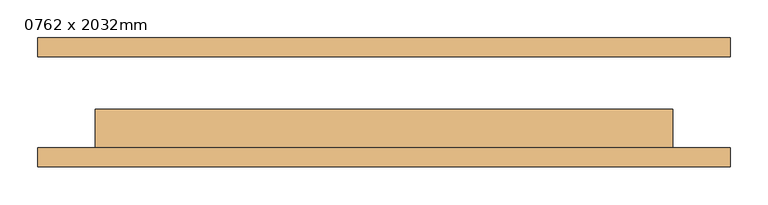
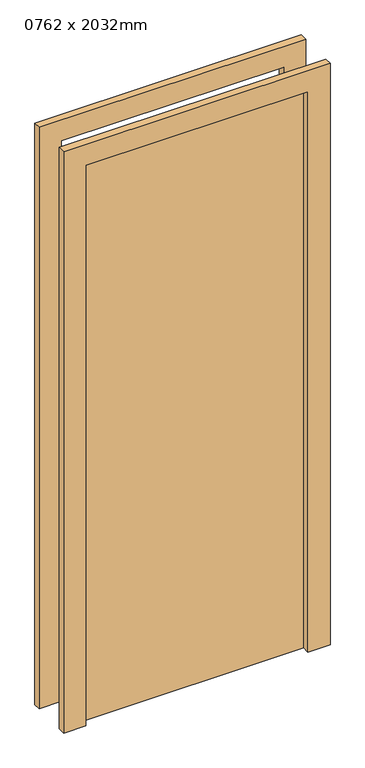
"""IFC4 building model written with IfcOpenShell, lengths in millimetres: door geometry, M_Folha única : 0762 x 2032mm."""

from ifc_helpers import new_model, si_unit, frame, origin, origin_with_axes, place, context, project, spatial, polyline, outline, extrude, source, transform, mapped, element, save


def door_0762_x_2032mm_5282416c(model_context):
    return source(origin(), model_context, "Body", "SweptSolid", [
        extrude(outline(polyline([(2108.0, -457.0), (0.0, -457.0), (0.0, -381.0), (2032.0, -381.0), (2032.0, 381.0), (0.0, 381.0), (0.0, 457.0), (2108.0, 457.0), (2108.0, -457.0)])), frame((0.0, -85.0, 0.0), z_axis=(0.0, 1.0, 0.0), x_axis=(0.0, 0.0, 1.0)), (0.0, 0.0, 1.0), 25.0),
        extrude(outline(polyline([(2108.0, 457.0), (2108.0, -457.0), (0.0, -457.0), (0.0, -381.0), (2032.0, -381.0), (2032.0, 381.0), (0.0, 381.0), (0.0, 457.0), (2108.0, 457.0)])), frame((0.0, 60.0, 0.0), z_axis=(0.0, 1.0, 0.0), x_axis=(0.0, 0.0, 1.0)), (0.0, 0.0, 1.0), 25.0),
        extrude(outline(polyline([(381.0, -9.0), (381.0, -60.0), (-381.0, -60.0), (-381.0, -9.0), (381.0, -9.0)])), origin_with_axes(), (0.0, 0.0, 1.0), 2032.0),
    ])


if __name__ == "__main__":
    model = new_model("IFC4")
    model_context = context("Model", 3, world=origin())
    ifc_project = project(units=[si_unit("LENGTHUNIT", "METRE", prefix="MILLI")], contexts=[model_context])
    site = spatial("IfcSite", under=ifc_project)
    building = spatial("IfcBuilding", under=site)
    placement = place(None, origin())
    door_0762_x_2032mm_shape = door_0762_x_2032mm_5282416c(model_context)
    element("IfcDoor", 1, ObjectType="M_Folha única : 0762 x 2032mm", at=placement, inside=building, context=model_context, shape_type="MappedRepresentation", body=[
        mapped(door_0762_x_2032mm_shape, transform((0.0, 0.0, 0.0), x_axis=(1.0, 0.0, 0.0), y_axis=(0.0, 1.0, 0.0), z_axis=(0.0, 0.0, 1.0))),
    ])
    save(model, "model.ifc")

# Revit data of these elements
# Type "M_Folha única : 0762 x 2032mm"
#   Type Mark = "28"
#   Construction Type Id = "MDOOR"
#   Analytic Construction = "Metal"
#   Thickness = 0.051 m
#   Thermal Resistance (R) = 0.270117 (m²·K)/W
#   Heat Transfer Coefficient (U) = 3.7021 W/(m²·K)
#   Height = 2.032 m
#   Projeção da apara externa = 0.025 m
#   Projeção da apara interna = 0.025 m
#   Largura da apara = 0.076 m
#   Width = 0.762 m
#   Define Thermal Properties by = 1
#   Define Thermal Properties by = 1
#   Material da porta = Porta - Painel
#   Material da moldura = Porta - Batente
#   Visual Light Transmittance = 0
#   Solar Heat Gain Coefficient = 0
#   Function = (empty or 0)
#   Wall Closure = (empty or 0)
# Element 1 (IfcDoor, "M_Folha única : 0762 x 2032mm")
#   Materials on its faces: "Porta - Batente", "Porta - Painel"
# Materials
#   "Porta - Painel": class "Madeira", colour RGB 210 159 95, transparency 0, Cost = 0
#   "Porta - Batente": class "Diversos", colour RGB 118 70 51, transparency 0, Cost = 0
